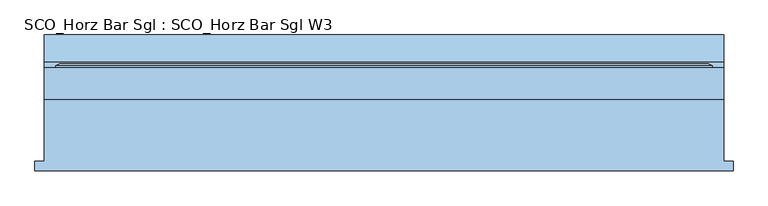
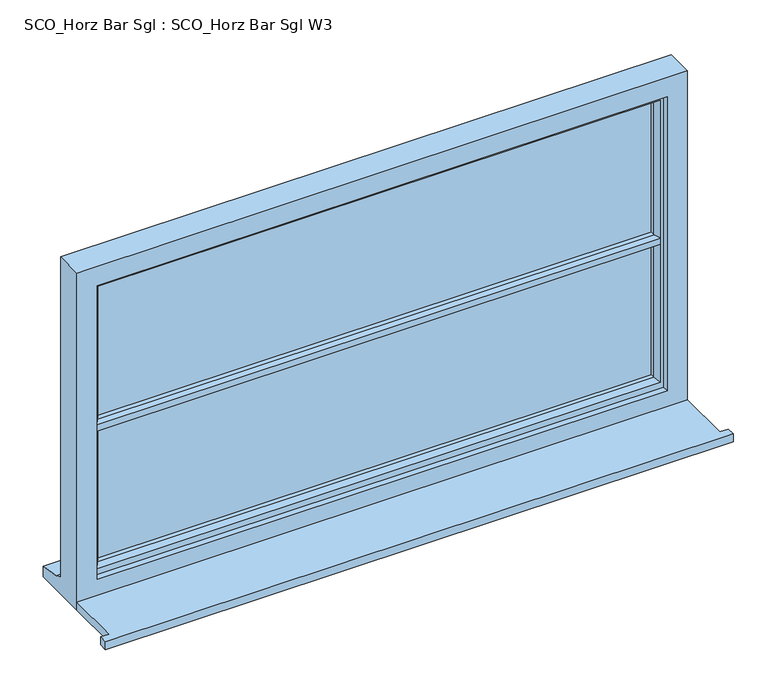
"""IFC4 building model written with IfcOpenShell, lengths in millimetres: window geometry, SCO_Horz Bar Sgl : SCO_Horz Bar Sgl W3."""

from ifc_helpers import new_model, si_unit, frame, origin, place, context, project, spatial, polyline, outline, extrude, faceted_brep, source, transform, mapped, element, save


def sco_horz_bar_sgl_sco_horz_bar_sgl_w3_c0565045(model_context):
    return source(origin(), model_context, "Body", "SolidModel", [
        extrude(outline(polyline([(-925.0, -191.5434322), (-925.0, -166.5434322), (-900.0, -166.5434322), (-900.0, -2.0434322), (900.0, -2.0434322), (900.0, -166.5434322), (925.0, -166.5434322), (925.0, -191.5434322), (-925.0, -191.5434322)])), frame((0.0, 0.0, 1060.0), z_axis=(0.0, 0.0, 1.0), x_axis=(1.0, 0.0, 0.0)), (0.0, 0.0, 1.0), 25.0),
        faceted_brep([(-900.0, -2.0434322, 1060.0), (900.0, -2.0434322, 1060.0), (900.0, -2.0434322, 2110.0), (-900.0, -2.0434322, 2110.0), (-840.0, -2.0434322, 2050.0), (840.0, -2.0434322, 2050.0), (840.0, -2.0434322, 1135.0), (-840.0, -2.0434322, 1135.0), (-900.0, 80.9565678, 2110.0), (-900.0, 80.9565678, 1111.0), (-900.0, 95.9565678, 1109.68767), (-900.0, 95.9565678, 1104.7449676), (-900.0, 168.4565678, 1093.8088847), (-900.0, 168.4565678, 1060.0), (900.0, 80.9565678, 2110.0), (900.0, 80.9565678, 1111.0), (-860.0, 80.9565678, 2070.0), (-860.0, 80.9565678, 1123.0), (860.0, 80.9565678, 1123.0), (860.0, 80.9565678, 2070.0), (-860.0, 15.9565678, 2070.0), (-860.0, 15.9565678, 1123.0), (860.0, 15.9565678, 2070.0), (860.0, 15.9565678, 1123.0), (-840.0, 15.9565678, 2050.0), (-840.0, 15.9565678, 1135.0), (840.0, 15.9565678, 1135.0), (840.0, 15.9565678, 2050.0), (900.0, 168.4565678, 1060.0), (900.0, 168.4565678, 1093.8088847), (900.0, 95.9565678, 1104.7449676), (900.0, 95.9565678, 1109.68767)], [[[0, 1, 2, 3], [4, 5, 6, 7]], [[0, 3, 8, 9, 10, 11, 12, 13]], [[9, 8, 14, 15], [16, 17, 18, 19]], [[17, 16, 20, 21]], [[20, 22, 23, 21], [24, 25, 26, 27]], [[24, 4, 7, 25]], [[3, 2, 14, 8]], [[16, 19, 22, 20]], [[5, 4, 24, 27]], [[15, 14, 2, 1, 28, 29, 30, 31]], [[19, 18, 23, 22]], [[5, 27, 26, 6]], [[28, 1, 0, 13]], [[29, 28, 13, 12]], [[30, 29, 12, 11]], [[31, 30, 11, 10]], [[15, 31, 10, 9]], [[21, 23, 18, 17]], [[7, 6, 26, 25]]]),
        extrude(outline(polyline([(830.1480377, 44.9565678), (-830.0, 44.9565678), (-830.0, 68.9565678), (830.1480377, 68.9565678), (830.1480377, 44.9565678)])), frame((0.0, 0.0, 1153.0), z_axis=(0.0, 0.0, 1.0), x_axis=(1.0, 0.0, 0.0)), (0.0, 0.0, 1.0), 434.3307627),
        extrude(outline(polyline([(830.1480377, 44.9565678), (-830.0, 44.9565678), (-830.0, 68.9565678), (830.1480377, 68.9565678), (830.1480377, 44.9565678)])), frame((0.0, 0.0, 1597.6692373), z_axis=(0.0, 0.0, 1.0), x_axis=(1.0, 0.0, 0.0)), (0.0, 0.0, 1.0), 442.3307627),
        extrude(outline(polyline([(92.5035732, 1597.6692373), (92.5035732, 1587.3307627), (86.8277797, 1577.5), (68.9565678, 1577.5), (68.9565678, 1584.5), (44.9565678, 1584.5), (44.9565678, 1577.5), (30.4494677, 1577.5), (15.9565678, 1582.6480377), (15.9565678, 1602.3519623), (30.4494677, 1607.5), (44.9565678, 1607.5), (44.9565678, 1600.5), (68.9565678, 1600.5), (68.9565678, 1607.5), (86.8277797, 1607.5), (92.5035732, 1597.6692373)])), frame((-830.1480377, 0.0, 0.0), z_axis=(1.0, 0.0, 0.0), x_axis=(0.0, 1.0, 0.0)), (0.0, 0.0, 1.0), 1660.2960754),
        faceted_brep([(-870.0, 80.9565678, 2072.0), (-870.0, 86.7300705, 2072.0), (-870.0, 86.7300705, 1113.0), (-870.0, 80.9565678, 1113.0), (-860.0, 15.9565678, 2062.0), (-860.0, 80.9565678, 2062.0), (-860.0, 80.9565678, 1123.0), (-860.0, 15.9565678, 1123.0), (-820.0, 30.4494677, 2022.0), (-830.1480377, 15.9565678, 2032.1480377), (-830.1480377, 15.9565678, 1152.8519623), (-820.0, 30.4494677, 1163.0), (-820.0, 44.9565678, 2022.0), (-820.0, 44.9565678, 1163.0), (-830.0, 68.9565678, 2032.0), (-830.0, 44.9565678, 2032.0), (-830.0, 44.9565678, 1153.0), (-830.0, 68.9565678, 1153.0), (-820.0, 86.7300705, 2022.0), (-820.0, 68.9565678, 2022.0), (-820.0, 68.9565678, 1163.0), (-820.0, 86.7300705, 1163.0), (-830.0, 92.5035732, 2032.0), (-830.0, 92.5035732, 1153.0), (-859.2153903, 92.5035732, 2061.2153903), (-859.2153903, 92.5035732, 1123.7846097), (870.0, 86.7300705, 1113.0), (870.0, 80.9565678, 1113.0), (860.0, 80.9565678, 1123.0), (860.0, 15.9565678, 1123.0), (830.1480377, 15.9565678, 1152.8519623), (820.0, 30.4494677, 1163.0), (820.0, 44.9565678, 1163.0), (830.0, 44.9565678, 1153.0), (830.0, 68.9565678, 1153.0), (820.0, 68.9565678, 1163.0), (820.0, 86.7300705, 1163.0), (830.0, 92.5035732, 1153.0), (859.2153903, 92.5035732, 1123.7846097), (870.0, 86.7300705, 2072.0), (870.0, 80.9565678, 2072.0), (860.0, 80.9565678, 2062.0), (860.0, 15.9565678, 2062.0), (830.1480377, 15.9565678, 2032.1480377), (820.0, 30.4494677, 2022.0), (820.0, 44.9565678, 2022.0), (830.0, 44.9565678, 2032.0), (830.0, 68.9565678, 2032.0), (820.0, 68.9565678, 2022.0), (820.0, 86.7300705, 2022.0), (830.0, 92.5035732, 2032.0), (859.2153903, 92.5035732, 2061.2153903)], [[[0, 1, 2, 3]], [[4, 5, 6, 7]], [[8, 9, 10, 11]], [[12, 8, 11, 13]], [[14, 15, 16, 17]], [[18, 19, 20, 21]], [[22, 18, 21, 23]], [[1, 24, 25, 2]], [[3, 2, 26, 27]], [[7, 6, 28, 29]], [[11, 10, 30, 31]], [[13, 11, 31, 32]], [[17, 16, 33, 34]], [[21, 20, 35, 36]], [[23, 21, 36, 37]], [[2, 25, 38, 26]], [[27, 26, 39, 40]], [[29, 28, 41, 42]], [[31, 30, 43, 44]], [[32, 31, 44, 45]], [[34, 33, 46, 47]], [[36, 35, 48, 49]], [[37, 36, 49, 50]], [[26, 38, 51, 39]], [[40, 39, 1, 0]], [[3, 27, 40, 0], [5, 41, 28, 6]], [[42, 41, 5, 4]], [[7, 29, 42, 4], [9, 43, 30, 10]], [[44, 43, 9, 8]], [[45, 44, 8, 12]], [[15, 46, 33, 16], [13, 32, 45, 12]], [[47, 46, 15, 14]], [[17, 34, 47, 14], [19, 48, 35, 20]], [[49, 48, 19, 18]], [[50, 49, 18, 22]], [[24, 51, 38, 25], [23, 37, 50, 22]], [[39, 51, 24, 1]]]),
    ])


if __name__ == "__main__":
    model = new_model("IFC4")
    model_context = context("Model", 3, world=origin())
    ifc_project = project(units=[si_unit("LENGTHUNIT", "METRE", prefix="MILLI")], contexts=[model_context])
    site = spatial("IfcSite", under=ifc_project)
    building = spatial("IfcBuilding", under=site)
    placement = place(None, origin())
    sco_horz_bar_sgl_sco_horz_bar_sgl_w3_shape = sco_horz_bar_sgl_sco_horz_bar_sgl_w3_c0565045(model_context)
    element("IfcWindow", 1, ObjectType="SCO_Horz Bar Sgl : SCO_Horz Bar Sgl W3", at=placement, inside=building, context=model_context, shape_type="MappedRepresentation", body=[
        mapped(sco_horz_bar_sgl_sco_horz_bar_sgl_w3_shape, transform((0.0, 0.0, 0.0), x_axis=(1.0, 0.0, 0.0), y_axis=(0.0, 1.0, 0.0), z_axis=(0.0, 0.0, 1.0))),
    ])
    save(model, "model.ifc")

# Revit data of these elements
# Type "SCO_Horz Bar Sgl : SCO_Horz Bar Sgl W3"
#   Type Mark = "W3"
#   Operation = "SinglePanel"
#   Manufacturer = "Revit"
#   Keynote = "L10"
#   Wrap Layers (Ext) from Ext = 102.5 mm
#   Wrap Layers (Int) from Ext = 177.5 mm
#   Window Board Projection = 25 mm
#   Window Board Extension = 25 mm
#   Rough Width = 1800 mm
#   Rough Height = 1050 mm
#   Height = 1050 mm
#   Width = 1800 mm
#   Glazing Thickness = 24 mm
#   FrameOffset - External = 102.5 mm
#   Frame Depth = 65 mm
#   Ext Leaf Thickness (Scot) = 102.5 mm
#   Ext Leaf Overlap (Scot) = 25 mm
#   Default Head Height = 2110 mm
#   Cill Depth = 87.5 mm
#   Cavity Closer Width = 50 mm
#   Cavity Closer Offset from Ext = 102.5 mm
#   Cavity Closer Depth = 85 mm
#   Vis - Cavity Closers = yes
#   Material Trim = Window Frame
#   Material Glass = Glass
#   Material Frame = Window Frame
#   Wall Closure = (empty or 0)
# Element 1 (IfcWindow, "SCO_Horz Bar Sgl : SCO_Horz Bar Sgl W3")
#   Materials on its faces: "Window Frame", "Glass"
# Materials
#   "Window Frame": class "Miscellaneous", colour RGB 249 249 249, transparency 0
#   "Glass": class "Glass", colour RGB 0 128 192, transparency 0.75
